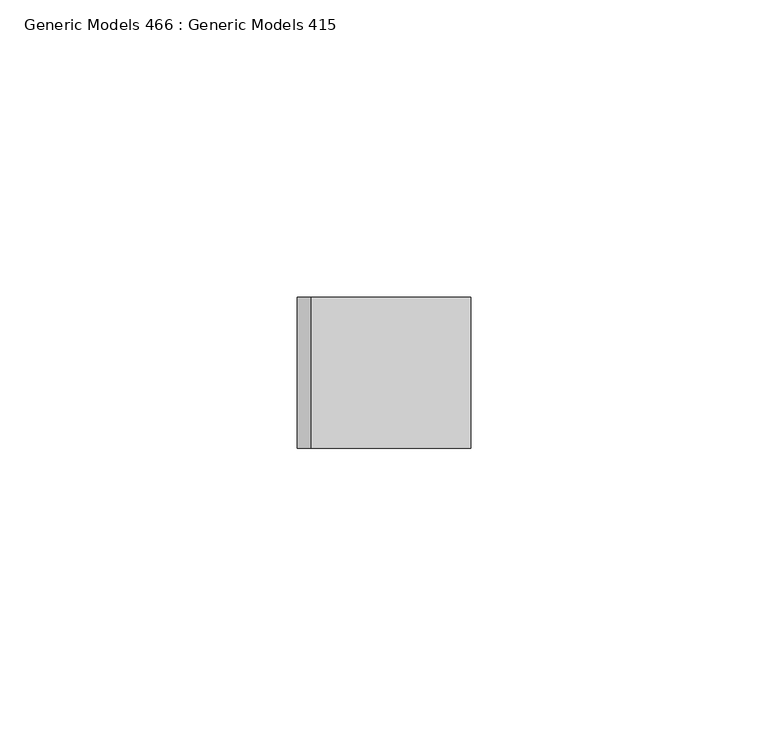
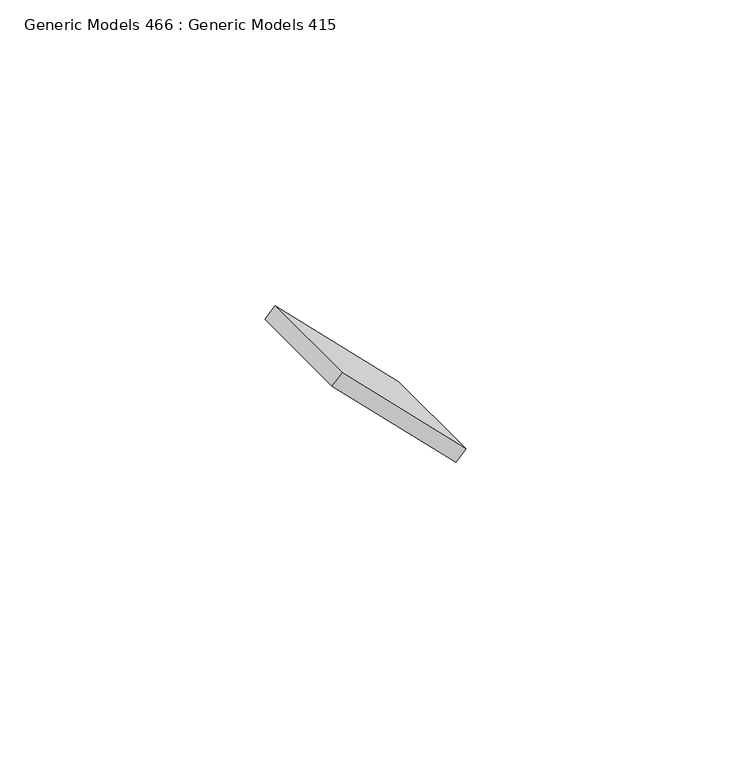
"""IFC4 building model written with IfcOpenShell, lengths in millimetres: proxy geometry, Generic Models 466 : Generic Models 415."""

from ifc_helpers import new_model, si_unit, frame, origin, place, context, project, spatial, polyline, outline, extrude, source, transform, mapped, element, save


def generic_models_466_generic_models_415_654adb48(model_context):
    return source(origin(), model_context, "Body", "SweptSolid", [
        extrude(outline(polyline([(0.0, -38.1), (0.0, 0.0), (25.4, 0.0), (25.4, -38.1), (0.0, -38.1)])), frame((-6869.8996186, -4475.9863946, 128289.5002957), z_axis=(0.7071067811864907, 0.0, 0.7071067811866044), x_axis=(0.0, -1.0, 0.0)), (0.0, 0.0, 1.0), 3.175),
    ])


if __name__ == "__main__":
    model = new_model("IFC4")
    model_context = context("Model", 3, world=origin())
    ifc_project = project(units=[si_unit("LENGTHUNIT", "METRE", prefix="MILLI")], contexts=[model_context])
    site = spatial("IfcSite", under=ifc_project)
    building = spatial("IfcBuilding", under=site)
    placement = place(None, origin())
    generic_models_466_generic_models_415_shape = generic_models_466_generic_models_415_654adb48(model_context)
    element("IfcBuildingElementProxy", 1, Name="Generic Models 466 : Generic Models 415", ObjectType="Generic Models 466 : Generic Models 415", at=placement, inside=building, context=model_context, shape_type="MappedRepresentation", body=[
        mapped(generic_models_466_generic_models_415_shape, transform((0.0, 0.0, 0.0), x_axis=(1.0, 0.0, 0.0), y_axis=(0.0, 1.0, 0.0), z_axis=(0.0, 0.0, 1.0))),
    ])
    save(model, "model.ifc")

# Revit data of these elements
# Element 1 (IfcBuildingElementProxy, "Generic Models 466 : Generic Models 415")
#   Materials on its faces: "_WELDED STEEL TABS FOR LOUVER ATTACHMENT"
# Materials
#   "_WELDED STEEL TABS FOR LOUVER ATTACHMENT": class "Metal", colour RGB 199 199 199, transparency 0, Description = "Structural steel 50ksi", Cost = 0
